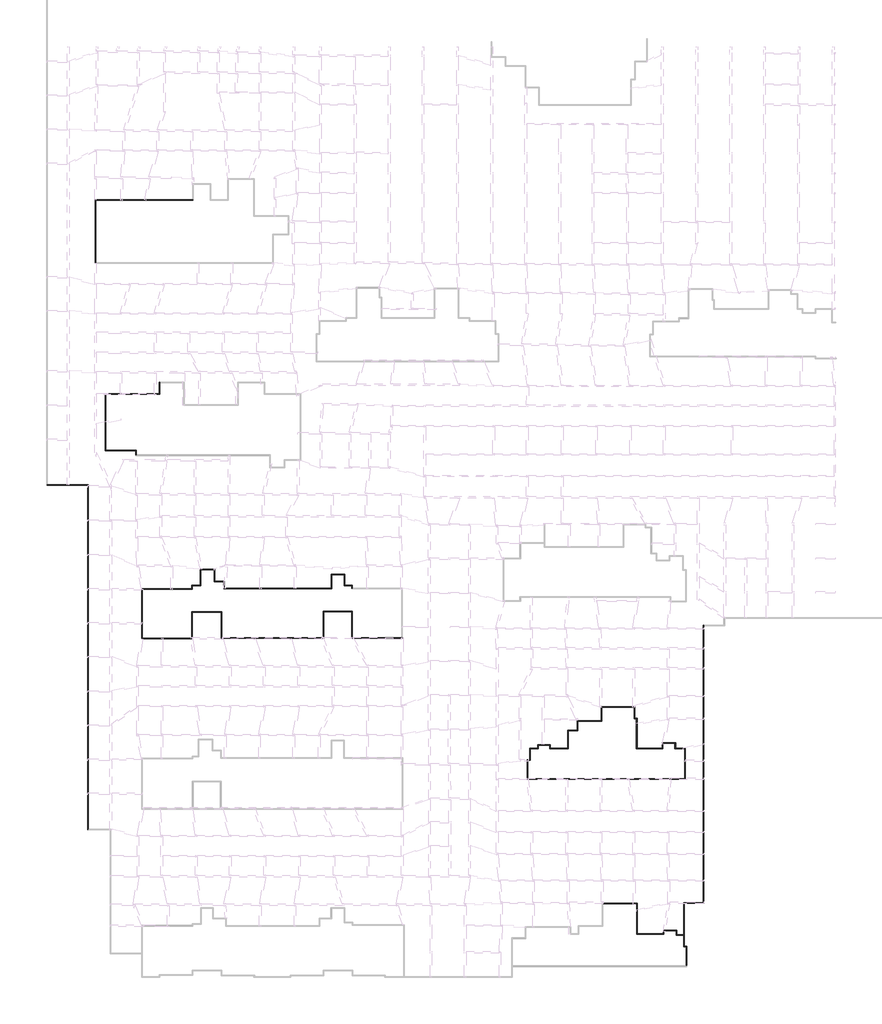
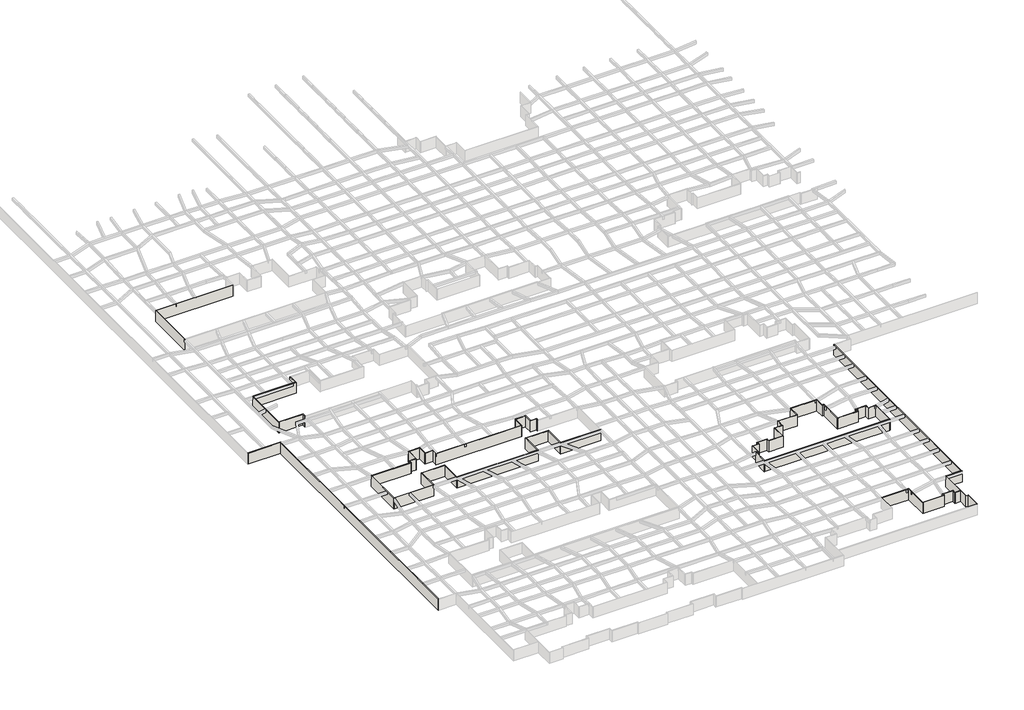
# One storey, part 2 of 45: 69 walls.
"""IFC4 building model written with IfcOpenShell, lengths in millimetres."""

from ifc_helpers import new_model, si_unit, origin, origin_with_axes, place, context, project, spatial, polyline, outline, extrude, faceted_brep, element, save

model = new_model("IFC4")

# Units and contexts
model_context = context("Model", 3, world=origin())
ifc_project = project(units=[si_unit("LENGTHUNIT", "METRE", prefix="MILLI")], contexts=[model_context])

# Site, building, storey
site = spatial("IfcSite", under=ifc_project)
building = spatial("IfcBuilding", under=site)
storey = spatial("IfcBuildingStorey", under=building, Name="户型图", Elevation=0.0)

# Walls
placement = place(None, origin())
element("IfcWall", 1, ObjectType="所有墙体", at=placement, inside=storey, context=model_context, shape_type="Brep", body=[
    faceted_brep([(-154980.5216564, -79588.0123265, 0.0), (-145700.5216564, -79588.0123265, 0.0), (-145580.5216564, -79588.0123265, 0.0), (-145580.5216564, -79588.0123265, 3300.0), (-145700.5216564, -79588.0123265, 3300.0), (-154980.5216564, -79588.0123265, 3300.0), (-154980.5216564, -79468.0123265, 0.0), (-154980.5216564, -79468.0123265, 3300.0), (-145580.5216564, -79468.0123265, 3300.0), (-145580.5216564, -79468.0123265, 0.0)], [[[0, 1, 2, 3, 4, 5]], [[6, 7, 8, 9]], [[2, 1, 0, 6, 9]], [[5, 4, 3, 8, 7]], [[0, 5, 7, 6]], [[3, 2, 9, 8]]]),
])
element("IfcWall", 2, ObjectType="所有墙体", at=placement, inside=storey, context=model_context, shape_type="Brep", body=[
    faceted_brep([(-145700.5216564, -79588.0123265, 0.0), (-145700.5216564, -158288.0123265, 0.0), (-145700.5216564, -158288.0123265, 3300.0), (-145700.5216564, -79588.0123265, 3300.0), (-145580.5216564, -79588.0123265, 0.0), (-145580.5216564, -79588.0123265, 3300.0), (-145580.5216564, -158168.0123265, 3300.0), (-145580.5216564, -158288.0123265, 3300.0), (-145580.5216564, -158288.0123265, 0.0), (-145580.5216564, -158168.0123265, 0.0)], [[[0, 1, 2, 3]], [[4, 5, 6, 7, 8, 9]], [[1, 0, 4, 9, 8]], [[3, 2, 7, 6, 5]], [[0, 3, 5, 4]], [[2, 1, 8, 7]]]),
])
element("IfcWall", 3, ObjectType="所有墙体", at=placement, inside=storey, context=model_context, shape_type="Brep", body=[
    faceted_brep([(-8780.5216564, -189468.0123265, 0.0), (-8780.5216564, -184968.0123265, 0.0), (-8780.5216564, -184968.0123265, 3300.0), (-8780.5216564, -189468.0123265, 3300.0), (-8900.5216564, -189468.0123265, 0.0), (-8900.5216564, -189468.0123265, 3300.0), (-8900.5216564, -185088.0123265, 3300.0), (-8900.5216564, -184968.0123265, 3300.0), (-8900.5216564, -184968.0123265, 0.0), (-8900.5216564, -185088.0123265, 0.0)], [[[0, 1, 2, 3]], [[4, 5, 6, 7, 8, 9]], [[1, 0, 4, 9, 8]], [[3, 2, 7, 6, 5]], [[0, 3, 5, 4]], [[2, 1, 8, 7]]]),
])
element("IfcWall", 4, ObjectType="所有墙体", at=placement, inside=storey, context=model_context, shape_type="Brep", body=[
    faceted_brep([(-8900.5216564, -184968.0123265, 0.0), (-9380.5216564, -184968.0123265, 0.0), (-9500.5216564, -184968.0123265, 0.0), (-9500.5216564, -184968.0123265, 3300.0), (-9380.5216564, -184968.0123265, 3300.0), (-8900.5216564, -184968.0123265, 3300.0), (-8900.5216564, -185088.0123265, 0.0), (-8900.5216564, -185088.0123265, 3300.0), (-9500.5216564, -185088.0123265, 3300.0), (-9500.5216564, -185088.0123265, 0.0)], [[[0, 1, 2, 3, 4, 5]], [[6, 7, 8, 9]], [[2, 1, 0, 6, 9]], [[5, 4, 3, 8, 7]], [[0, 5, 7, 6]], [[3, 2, 9, 8]]]),
])
element("IfcWall", 5, ObjectType="所有墙体", at=placement, inside=storey, context=model_context, shape_type="Brep", body=[
    faceted_brep([(-9380.5216564, -184968.0123265, 0.0), (-9380.5216564, -175188.0123265, 0.0), (-9380.5216564, -175068.0123265, 0.0), (-9380.5216564, -175068.0123265, 3300.0), (-9380.5216564, -175188.0123265, 3300.0), (-9380.5216564, -184968.0123265, 3300.0), (-9500.5216564, -184968.0123265, 0.0), (-9500.5216564, -184968.0123265, 3300.0), (-9500.5216564, -182430.9342179, 3300.0), (-9500.5216564, -182310.9342179, 3300.0), (-9500.5216564, -175068.0123265, 3300.0), (-9500.5216564, -175068.0123265, 0.0), (-9500.5216564, -182310.9342179, 0.0), (-9500.5216564, -182430.9342179, 0.0)], [[[0, 1, 2, 3, 4, 5]], [[6, 7, 8, 9, 10, 11, 12, 13]], [[2, 1, 0, 6, 13, 12, 11]], [[5, 4, 3, 10, 9, 8, 7]], [[0, 5, 7, 6]], [[3, 2, 11, 10]]]),
])
element("IfcWall", 6, ObjectType="所有墙体", at=placement, inside=storey, context=model_context, shape_type="Brep", body=[
    faceted_brep([(-9380.5216564, -175188.0123265, 0.0), (-4880.5216564, -175188.0123265, 0.0), (-4880.5216564, -175188.0123265, 3300.0), (-9380.5216564, -175188.0123265, 3300.0), (-9380.5216564, -175068.0123265, 0.0), (-9380.5216564, -175068.0123265, 3300.0), (-5000.5216564, -175068.0123265, 3300.0), (-4880.5216564, -175068.0123265, 3300.0), (-4880.5216564, -175068.0123265, 0.0), (-5000.5216564, -175068.0123265, 0.0)], [[[0, 1, 2, 3]], [[4, 5, 6, 7, 8, 9]], [[1, 0, 4, 9, 8]], [[3, 2, 7, 6, 5]], [[0, 3, 5, 4]], [[2, 1, 8, 7]]]),
])
element("IfcWall", 7, ObjectType="所有墙体", at=placement, inside=storey, context=model_context, shape_type="Brep", body=[
    faceted_brep([(-4880.5216564, -175068.0123265, 0.0), (-4880.5216564, -111688.0123265, 0.0), (-4880.5216564, -111568.0123265, 0.0), (-4880.5216564, -111568.0123265, 3300.0), (-4880.5216564, -111688.0123265, 3300.0), (-4880.5216564, -175068.0123265, 3300.0), (-5000.5216564, -175068.0123265, 0.0), (-5000.5216564, -175068.0123265, 3300.0), (-5000.5216564, -111568.0123265, 3300.0), (-5000.5216564, -111568.0123265, 0.0)], [[[0, 1, 2, 3, 4, 5]], [[6, 7, 8, 9]], [[2, 1, 0, 6, 9]], [[5, 4, 3, 8, 7]], [[0, 5, 7, 6]], [[3, 2, 9, 8]]]),
])
element("IfcWall", 8, ObjectType="所有墙体", at=placement, inside=storey, context=model_context, shape_type="Brep", body=[
    faceted_brep([(-27951.0528269, -175221.8863426, 0.0), (-20271.0528269, -175221.8863426, 0.0), (-20151.0528269, -175221.8863426, 0.0), (-20151.0528269, -175221.8863426, 3300.0), (-20271.0528269, -175221.8863426, 3300.0), (-27951.0528269, -175221.8863426, 3300.0), (-27951.0528269, -175101.8863426, 0.0), (-27951.0528269, -175101.8863426, 3300.0), (-20151.0528269, -175101.8863426, 3300.0), (-20151.0528269, -175101.8863426, 0.0)], [[[0, 1, 2, 3, 4, 5]], [[6, 7, 8, 9]], [[2, 1, 0, 6, 9]], [[5, 4, 3, 8, 7]], [[0, 5, 7, 6]], [[3, 2, 9, 8]]]),
])
element("IfcWall", 9, ObjectType="所有墙体", at=placement, inside=storey, context=model_context, shape_type="Brep", body=[
    faceted_brep([(-20271.0528269, -175221.8863426, 0.0), (-20271.0528269, -182221.8863426, 0.0), (-20271.0528269, -182221.8863426, 3300.0), (-20271.0528269, -175221.8863426, 3300.0), (-20151.0528269, -175221.8863426, 0.0), (-20151.0528269, -175221.8863426, 3300.0), (-20151.0528269, -182101.8863426, 3300.0), (-20151.0528269, -182221.8863426, 3300.0), (-20151.0528269, -182221.8863426, 0.0), (-20151.0528269, -182101.8863426, 0.0)], [[[0, 1, 2, 3]], [[4, 5, 6, 7, 8, 9]], [[1, 0, 4, 9, 8]], [[3, 2, 7, 6, 5]], [[0, 3, 5, 4]], [[2, 1, 8, 7]]]),
])
element("IfcWall", 10, ObjectType="所有墙体", at=placement, inside=storey, context=model_context, shape_type="Brep", body=[
    faceted_brep([(-20151.0528269, -182221.8863426, 0.0), (-14051.0528269, -182221.8863426, 0.0), (-14051.0528269, -182221.8863426, 3300.0), (-20151.0528269, -182221.8863426, 3300.0), (-20151.0528269, -182101.8863426, 0.0), (-20151.0528269, -182101.8863426, 3300.0), (-14171.0528269, -182101.8863426, 3300.0), (-14051.0528269, -182101.8863426, 3300.0), (-14051.0528269, -182101.8863426, 0.0), (-14171.0528269, -182101.8863426, 0.0)], [[[0, 1, 2, 3]], [[4, 5, 6, 7, 8, 9]], [[1, 0, 4, 9, 8]], [[3, 2, 7, 6, 5]], [[0, 3, 5, 4]], [[2, 1, 8, 7]]]),
])
element("IfcWall", 11, ObjectType="所有墙体", at=placement, inside=storey, context=model_context, shape_type="Brep", body=[
    faceted_brep([(-14051.0528269, -182101.8863426, 0.0), (-14051.0528269, -181430.9342179, 0.0), (-14051.0528269, -181310.9342179, 0.0), (-14051.0528269, -181310.9342179, 3300.0), (-14051.0528269, -181430.9342179, 3300.0), (-14051.0528269, -182101.8863426, 3300.0), (-14171.0528269, -182101.8863426, 0.0), (-14171.0528269, -182101.8863426, 3300.0), (-14171.0528269, -181310.9342179, 3300.0), (-14171.0528269, -181310.9342179, 0.0)], [[[0, 1, 2, 3, 4, 5]], [[6, 7, 8, 9]], [[2, 1, 0, 6, 9]], [[5, 4, 3, 8, 7]], [[0, 5, 7, 6]], [[3, 2, 9, 8]]]),
])
element("IfcWall", 12, ObjectType="所有墙体", at=placement, inside=storey, context=model_context, shape_type="Brep", body=[
    faceted_brep([(-14051.0528269, -181430.9342179, 0.0), (-11171.0528269, -181430.9342179, 0.0), (-11051.0528269, -181430.9342179, 0.0), (-11051.0528269, -181430.9342179, 3300.0), (-11171.0528269, -181430.9342179, 3300.0), (-14051.0528269, -181430.9342179, 3300.0), (-14051.0528269, -181310.9342179, 0.0), (-14051.0528269, -181310.9342179, 3300.0), (-11051.0528269, -181310.9342179, 3300.0), (-11051.0528269, -181310.9342179, 0.0)], [[[0, 1, 2, 3, 4, 5]], [[6, 7, 8, 9]], [[2, 1, 0, 6, 9]], [[5, 4, 3, 8, 7]], [[0, 5, 7, 6]], [[3, 2, 9, 8]]]),
])
element("IfcWall", 13, ObjectType="所有墙体", at=placement, inside=storey, context=model_context, shape_type="Brep", body=[
    faceted_brep([(-11171.0528269, -181430.9342179, 0.0), (-11171.0528269, -182430.9342179, 0.0), (-11171.0528269, -182430.9342179, 3300.0), (-11171.0528269, -181430.9342179, 3300.0), (-11051.0528269, -181430.9342179, 0.0), (-11051.0528269, -181430.9342179, 3300.0), (-11051.0528269, -182310.9342179, 3300.0), (-11051.0528269, -182430.9342179, 3300.0), (-11051.0528269, -182430.9342179, 0.0), (-11051.0528269, -182310.9342179, 0.0)], [[[0, 1, 2, 3]], [[4, 5, 6, 7, 8, 9]], [[1, 0, 4, 9, 8]], [[3, 2, 7, 6, 5]], [[0, 3, 5, 4]], [[2, 1, 8, 7]]]),
])
element("IfcWall", 14, ObjectType="所有墙体", at=placement, inside=storey, context=model_context, shape_type="SweptSolid", body=[
    extrude(outline(polyline([(-9500.5216564, -182430.9342179), (-11051.0528269, -182430.9342179), (-11051.0528269, -182310.9342179), (-9500.5216564, -182310.9342179), (-9500.5216564, -182430.9342179)])), origin_with_axes(), (0.0, 0.0, 1.0), 3300.0),
])
element("IfcWall", 15, ObjectType="所有墙体", at=placement, inside=storey, context=model_context, shape_type="Brep", body=[
    faceted_brep([(-133310.9438267, -103315.0953667, 0.0), (-133310.9438267, -114643.3262311, 0.0), (-133310.9438267, -114643.3262311, 3300.0), (-133310.9438267, -103315.0953667, 3300.0), (-133190.9438267, -103315.0953667, 0.0), (-133190.9438267, -103315.0953667, 3300.0), (-133190.9438267, -103435.0953667, 3300.0), (-133190.9438267, -114523.3262311, 3300.0), (-133190.9438267, -114643.3262311, 3300.0), (-133190.9438267, -114643.3262311, 0.0), (-133190.9438267, -114523.3262311, 0.0), (-133190.9438267, -103435.0953667, 0.0)], [[[0, 1, 2, 3]], [[4, 5, 6, 7, 8, 9, 10, 11]], [[1, 0, 4, 11, 10, 9]], [[3, 2, 8, 7, 6, 5]], [[2, 1, 9, 8]], [[0, 3, 5, 4]]]),
])
element("IfcWall", 16, ObjectType="所有墙体", at=placement, inside=storey, context=model_context, shape_type="Brep", body=[
    faceted_brep([(-133190.9438267, -114643.3262311, 0.0), (-121790.9438267, -114643.3262311, 0.0), (-121790.9438267, -114643.3262311, 3300.0), (-133190.9438267, -114643.3262311, 3300.0), (-133190.9438267, -114523.3262311, 0.0), (-133190.9438267, -114523.3262311, 3300.0), (-121910.9438267, -114523.3262311, 3300.0), (-121790.9438267, -114523.3262311, 3300.0), (-121790.9438267, -114523.3262311, 0.0), (-121910.9438267, -114523.3262311, 0.0)], [[[0, 1, 2, 3]], [[4, 5, 6, 7, 8, 9]], [[1, 0, 4, 9, 8]], [[3, 2, 7, 6, 5]], [[0, 3, 5, 4]], [[2, 1, 8, 7]]]),
])
element("IfcWall", 17, ObjectType="所有墙体", at=placement, inside=storey, context=model_context, shape_type="Brep", body=[
    faceted_brep([(-121790.9438267, -114523.3262311, 0.0), (-121790.9438267, -108643.3262311, 0.0), (-121790.9438267, -108523.3262311, 0.0), (-121790.9438267, -108523.3262311, 3300.0), (-121790.9438267, -108643.3262311, 3300.0), (-121790.9438267, -114523.3262311, 3300.0), (-121910.9438267, -114523.3262311, 0.0), (-121910.9438267, -114523.3262311, 3300.0), (-121910.9438267, -108523.3262311, 3300.0), (-121910.9438267, -108523.3262311, 0.0)], [[[0, 1, 2, 3, 4, 5]], [[6, 7, 8, 9]], [[2, 1, 0, 6, 9]], [[5, 4, 3, 8, 7]], [[0, 5, 7, 6]], [[3, 2, 9, 8]]]),
])
element("IfcWall", 18, ObjectType="所有墙体", at=placement, inside=storey, context=model_context, shape_type="Brep", body=[
    faceted_brep([(-121790.9438267, -108643.3262311, 0.0), (-115210.9438267, -108643.3262311, 0.0), (-115090.9438267, -108643.3262311, 0.0), (-115090.9438267, -108643.3262311, 3300.0), (-115210.9438267, -108643.3262311, 3300.0), (-121790.9438267, -108643.3262311, 3300.0), (-121790.9438267, -108523.3262311, 0.0), (-121790.9438267, -108523.3262311, 3300.0), (-115090.9438267, -108523.3262311, 3300.0), (-115090.9438267, -108523.3262311, 0.0)], [[[0, 1, 2, 3, 4, 5]], [[6, 7, 8, 9]], [[2, 1, 0, 6, 9]], [[5, 4, 3, 8, 7]], [[0, 5, 7, 6]], [[3, 2, 9, 8]]]),
])
element("IfcWall", 19, ObjectType="所有墙体", at=placement, inside=storey, context=model_context, shape_type="Brep", body=[
    faceted_brep([(-115210.9438267, -108643.3262311, 0.0), (-115210.9438267, -114616.2273817, 0.0), (-115210.9438267, -114616.2273817, 3300.0), (-115210.9438267, -108643.3262311, 3300.0), (-115090.9438267, -108643.3262311, 0.0), (-115090.9438267, -108643.3262311, 3300.0), (-115090.9438267, -114496.2273817, 3300.0), (-115090.9438267, -114616.2273817, 3300.0), (-115090.9438267, -114616.2273817, 0.0), (-115090.9438267, -114496.2273817, 0.0)], [[[0, 1, 2, 3]], [[4, 5, 6, 7, 8, 9]], [[1, 0, 4, 9, 8]], [[3, 2, 7, 6, 5]], [[0, 3, 5, 4]], [[2, 1, 8, 7]]]),
])
element("IfcWall", 20, ObjectType="所有墙体", at=placement, inside=storey, context=model_context, shape_type="Brep", body=[
    faceted_brep([(-115090.9438267, -114616.2273817, 0.0), (-91790.9438267, -114616.2273817, 0.0), (-91790.9438267, -114616.2273817, 3300.0), (-115090.9438267, -114616.2273817, 3300.0), (-115090.9438267, -114496.2273817, 0.0), (-115090.9438267, -114496.2273817, 3300.0), (-91910.9438267, -114496.2273817, 3300.0), (-91790.9438267, -114496.2273817, 3300.0), (-91790.9438267, -114496.2273817, 0.0), (-91910.9438267, -114496.2273817, 0.0)], [[[0, 1, 2, 3]], [[4, 5, 6, 7, 8, 9]], [[1, 0, 4, 9, 8]], [[3, 2, 7, 6, 5]], [[0, 3, 5, 4]], [[2, 1, 8, 7]]]),
])
element("IfcWall", 21, ObjectType="所有墙体", at=placement, inside=storey, context=model_context, shape_type="Brep", body=[
    faceted_brep([(-91790.9438267, -114496.2273817, 0.0), (-91790.9438267, -108516.2273817, 0.0), (-91790.9438267, -108396.2273817, 0.0), (-91790.9438267, -108396.2273817, 3300.0), (-91790.9438267, -108516.2273817, 3300.0), (-91790.9438267, -114496.2273817, 3300.0), (-91910.9438267, -114496.2273817, 0.0), (-91910.9438267, -114496.2273817, 3300.0), (-91910.9438267, -108396.2273817, 3300.0), (-91910.9438267, -108396.2273817, 0.0)], [[[0, 1, 2, 3, 4, 5]], [[6, 7, 8, 9]], [[2, 1, 0, 6, 9]], [[5, 4, 3, 8, 7]], [[0, 5, 7, 6]], [[3, 2, 9, 8]]]),
])
element("IfcWall", 22, ObjectType="所有墙体", at=placement, inside=storey, context=model_context, shape_type="Brep", body=[
    faceted_brep([(-91790.9438267, -108516.2273817, 0.0), (-85410.9438267, -108516.2273817, 0.0), (-85290.9438267, -108516.2273817, 0.0), (-85290.9438267, -108516.2273817, 3300.0), (-85410.9438267, -108516.2273817, 3300.0), (-91790.9438267, -108516.2273817, 3300.0), (-91790.9438267, -108396.2273817, 0.0), (-91790.9438267, -108396.2273817, 3300.0), (-85290.9438267, -108396.2273817, 3300.0), (-85290.9438267, -108396.2273817, 0.0)], [[[0, 1, 2, 3, 4, 5]], [[6, 7, 8, 9]], [[2, 1, 0, 6, 9]], [[5, 4, 3, 8, 7]], [[0, 5, 7, 6]], [[3, 2, 9, 8]]]),
])
element("IfcWall", 23, ObjectType="所有墙体", at=placement, inside=storey, context=model_context, shape_type="Brep", body=[
    faceted_brep([(-85410.9438267, -108516.2273817, 0.0), (-85410.9438267, -114616.2273817, 0.0), (-85410.9438267, -114616.2273817, 3300.0), (-85410.9438267, -108516.2273817, 3300.0), (-85290.9438267, -108516.2273817, 0.0), (-85290.9438267, -108516.2273817, 3300.0), (-85290.9438267, -114496.2273817, 3300.0), (-85290.9438267, -114616.2273817, 3300.0), (-85290.9438267, -114616.2273817, 0.0), (-85290.9438267, -114496.2273817, 0.0)], [[[0, 1, 2, 3]], [[4, 5, 6, 7, 8, 9]], [[1, 0, 4, 9, 8]], [[3, 2, 7, 6, 5]], [[0, 3, 5, 4]], [[2, 1, 8, 7]]]),
])
element("IfcWall", 24, ObjectType="所有墙体", at=placement, inside=storey, context=model_context, shape_type="Brep", body=[
    faceted_brep([(-85290.9438267, -114616.2273817, 0.0), (-73790.9438267, -114616.2273817, 0.0), (-73790.9438267, -114616.2273817, 3300.0), (-85290.9438267, -114616.2273817, 3300.0), (-85290.9438267, -114496.2273817, 0.0), (-85290.9438267, -114496.2273817, 3300.0), (-73910.9438267, -114496.2273817, 3300.0), (-73790.9438267, -114496.2273817, 3300.0), (-73790.9438267, -114496.2273817, 0.0), (-73910.9438267, -114496.2273817, 0.0)], [[[0, 1, 2, 3]], [[4, 5, 6, 7, 8, 9]], [[1, 0, 4, 9, 8]], [[3, 2, 7, 6, 5]], [[0, 3, 5, 4]], [[2, 1, 8, 7]]]),
])
element("IfcWall", 25, ObjectType="所有墙体", at=placement, inside=storey, context=model_context, shape_type="Brep", body=[
    faceted_brep([(-85290.9438267, -103096.2273817, 0.0), (-85290.9438267, -102496.2273817, 0.0), (-85290.9438267, -102496.2273817, 3300.0), (-85290.9438267, -103096.2273817, 3300.0), (-85410.9438267, -103096.2273817, 0.0), (-85410.9438267, -103096.2273817, 3300.0), (-85410.9438267, -102616.2273817, 3300.0), (-85410.9438267, -102496.2273817, 3300.0), (-85410.9438267, -102496.2273817, 0.0), (-85410.9438267, -102616.2273817, 0.0)], [[[0, 1, 2, 3]], [[4, 5, 6, 7, 8, 9]], [[1, 0, 4, 9, 8]], [[3, 2, 7, 6, 5]], [[0, 3, 5, 4]], [[2, 1, 8, 7]]]),
])
element("IfcWall", 26, ObjectType="所有墙体", at=placement, inside=storey, context=model_context, shape_type="Brep", body=[
    faceted_brep([(-85410.9438267, -102496.2273817, 0.0), (-86990.9438267, -102496.2273817, 0.0), (-87110.9438267, -102496.2273817, 0.0), (-87110.9438267, -102496.2273817, 3300.0), (-86990.9438267, -102496.2273817, 3300.0), (-85410.9438267, -102496.2273817, 3300.0), (-85410.9438267, -102616.2273817, 0.0), (-85410.9438267, -102616.2273817, 3300.0), (-87110.9438267, -102616.2273817, 3300.0), (-87110.9438267, -102616.2273817, 0.0)], [[[0, 1, 2, 3, 4, 5]], [[6, 7, 8, 9]], [[2, 1, 0, 6, 9]], [[5, 4, 3, 8, 7]], [[0, 5, 7, 6]], [[3, 2, 9, 8]]]),
])
element("IfcWall", 27, ObjectType="所有墙体", at=placement, inside=storey, context=model_context, shape_type="Brep", body=[
    faceted_brep([(-86990.9438267, -102496.2273817, 0.0), (-86990.9438267, -99996.2273817, 0.0), (-86990.9438267, -99996.2273817, 3300.0), (-86990.9438267, -102496.2273817, 3300.0), (-87110.9438267, -102496.2273817, 0.0), (-87110.9438267, -102496.2273817, 3300.0), (-87110.9438267, -100116.2273817, 3300.0), (-87110.9438267, -99996.2273817, 3300.0), (-87110.9438267, -99996.2273817, 0.0), (-87110.9438267, -100116.2273817, 0.0)], [[[0, 1, 2, 3]], [[4, 5, 6, 7, 8, 9]], [[1, 0, 4, 9, 8]], [[3, 2, 7, 6, 5]], [[0, 3, 5, 4]], [[2, 1, 8, 7]]]),
])
element("IfcWall", 28, ObjectType="所有墙体", at=placement, inside=storey, context=model_context, shape_type="Brep", body=[
    faceted_brep([(-87110.9438267, -99996.2273817, 0.0), (-90010.9438267, -99996.2273817, 0.0), (-90010.9438267, -99996.2273817, 3300.0), (-87110.9438267, -99996.2273817, 3300.0), (-87110.9438267, -100116.2273817, 0.0), (-87110.9438267, -100116.2273817, 3300.0), (-89890.9438267, -100116.2273817, 3300.0), (-90010.9438267, -100116.2273817, 3300.0), (-90010.9438267, -100116.2273817, 0.0), (-89890.9438267, -100116.2273817, 0.0)], [[[0, 1, 2, 3]], [[4, 5, 6, 7, 8, 9]], [[1, 0, 4, 9, 8]], [[3, 2, 7, 6, 5]], [[0, 3, 5, 4]], [[2, 1, 8, 7]]]),
])
element("IfcWall", 29, ObjectType="所有墙体", at=placement, inside=storey, context=model_context, shape_type="Brep", body=[
    faceted_brep([(-90010.9438267, -100116.2273817, 0.0), (-90010.9438267, -103096.2273817, 0.0), (-90010.9438267, -103216.2273817, 0.0), (-90010.9438267, -103216.2273817, 3300.0), (-90010.9438267, -103096.2273817, 3300.0), (-90010.9438267, -100116.2273817, 3300.0), (-89890.9438267, -100116.2273817, 0.0), (-89890.9438267, -100116.2273817, 3300.0), (-89890.9438267, -103216.2273817, 3300.0), (-89890.9438267, -103216.2273817, 0.0)], [[[0, 1, 2, 3, 4, 5]], [[6, 7, 8, 9]], [[2, 1, 0, 6, 9]], [[5, 4, 3, 8, 7]], [[0, 5, 7, 6]], [[3, 2, 9, 8]]]),
])
element("IfcWall", 30, ObjectType="所有墙体", at=placement, inside=storey, context=model_context, shape_type="Brep", body=[
    faceted_brep([(-90010.9438267, -103096.2273817, 0.0), (-114494.8894141, -103096.2273817, 0.0), (-114614.8894141, -103096.2273817, 0.0), (-114614.8894141, -103096.2273817, 3300.0), (-114494.8894141, -103096.2273817, 3300.0), (-90010.9438267, -103096.2273817, 3300.0), (-90010.9438267, -103216.2273817, 0.0), (-90010.9438267, -103216.2273817, 3300.0), (-114614.8894141, -103216.2273817, 3300.0), (-114614.8894141, -103216.2273817, 0.0)], [[[0, 1, 2, 3, 4, 5]], [[6, 7, 8, 9]], [[2, 1, 0, 6, 9]], [[5, 4, 3, 8, 7]], [[0, 5, 7, 6]], [[3, 2, 9, 8]]]),
])
element("IfcWall", 31, ObjectType="所有墙体", at=placement, inside=storey, context=model_context, shape_type="Brep", body=[
    faceted_brep([(-114494.8894141, -103096.2273817, 0.0), (-114494.8894141, -101496.2273817, 0.0), (-114494.8894141, -101496.2273817, 3300.0), (-114494.8894141, -103096.2273817, 3300.0), (-114614.8894141, -103096.2273817, 0.0), (-114614.8894141, -103096.2273817, 3300.0), (-114614.8894141, -101616.2273817, 3300.0), (-114614.8894141, -101496.2273817, 3300.0), (-114614.8894141, -101496.2273817, 0.0), (-114614.8894141, -101616.2273817, 0.0)], [[[0, 1, 2, 3]], [[4, 5, 6, 7, 8, 9]], [[1, 0, 4, 9, 8]], [[3, 2, 7, 6, 5]], [[0, 3, 5, 4]], [[2, 1, 8, 7]]]),
])
element("IfcWall", 32, ObjectType="所有墙体", at=placement, inside=storey, context=model_context, shape_type="Brep", body=[
    faceted_brep([(-114614.8894141, -101496.2273817, 0.0), (-116694.8894141, -101496.2273817, 0.0), (-116814.8894141, -101496.2273817, 0.0), (-116814.8894141, -101496.2273817, 3300.0), (-116694.8894141, -101496.2273817, 3300.0), (-114614.8894141, -101496.2273817, 3300.0), (-114614.8894141, -101616.2273817, 0.0), (-114614.8894141, -101616.2273817, 3300.0), (-116814.8894141, -101616.2273817, 3300.0), (-116814.8894141, -101616.2273817, 0.0)], [[[0, 1, 2, 3, 4, 5]], [[6, 7, 8, 9]], [[2, 1, 0, 6, 9]], [[5, 4, 3, 8, 7]], [[0, 5, 7, 6]], [[3, 2, 9, 8]]]),
])
element("IfcWall", 33, ObjectType="所有墙体", at=placement, inside=storey, context=model_context, shape_type="Brep", body=[
    faceted_brep([(-116694.8894141, -101496.2273817, 0.0), (-116694.8894141, -98815.2904885, 0.0), (-116694.8894141, -98815.2904885, 3300.0), (-116694.8894141, -101496.2273817, 3300.0), (-116814.8894141, -101496.2273817, 0.0), (-116814.8894141, -101496.2273817, 3300.0), (-116814.8894141, -98935.2904885, 3300.0), (-116814.8894141, -98815.2904885, 3300.0), (-116814.8894141, -98815.2904885, 0.0), (-116814.8894141, -98935.2904885, 0.0)], [[[0, 1, 2, 3]], [[4, 5, 6, 7, 8, 9]], [[1, 0, 4, 9, 8]], [[3, 2, 7, 6, 5]], [[0, 3, 5, 4]], [[2, 1, 8, 7]]]),
])
element("IfcWall", 34, ObjectType="所有墙体", at=placement, inside=storey, context=model_context, shape_type="Brep", body=[
    faceted_brep([(-116814.8894141, -98815.2904885, 0.0), (-120017.441353, -98815.2904885, 0.0), (-120017.441353, -98815.2904885, 3300.0), (-116814.8894141, -98815.2904885, 3300.0), (-116814.8894141, -98935.2904885, 0.0), (-116814.8894141, -98935.2904885, 3300.0), (-119897.441353, -98935.2904885, 3300.0), (-120017.441353, -98935.2904885, 3300.0), (-120017.441353, -98935.2904885, 0.0), (-119897.441353, -98935.2904885, 0.0)], [[[0, 1, 2, 3]], [[4, 5, 6, 7, 8, 9]], [[1, 0, 4, 9, 8]], [[3, 2, 7, 6, 5]], [[0, 3, 5, 4]], [[2, 1, 8, 7]]]),
])
element("IfcWall", 35, ObjectType="所有墙体", at=placement, inside=storey, context=model_context, shape_type="Brep", body=[
    faceted_brep([(-120017.441353, -98935.2904885, 0.0), (-120017.441353, -102496.2273817, 0.0), (-120017.441353, -102616.2273817, 0.0), (-120017.441353, -102616.2273817, 3300.0), (-120017.441353, -102496.2273817, 3300.0), (-120017.441353, -98935.2904885, 3300.0), (-119897.441353, -98935.2904885, 0.0), (-119897.441353, -98935.2904885, 3300.0), (-119897.441353, -102616.2273817, 3300.0), (-119897.441353, -102616.2273817, 0.0)], [[[0, 1, 2, 3, 4, 5]], [[6, 7, 8, 9]], [[2, 1, 0, 6, 9]], [[5, 4, 3, 8, 7]], [[0, 5, 7, 6]], [[3, 2, 9, 8]]]),
])
element("IfcWall", 36, ObjectType="所有墙体", at=placement, inside=storey, context=model_context, shape_type="Brep", body=[
    faceted_brep([(-120017.441353, -102496.2273817, 0.0), (-121910.9438267, -102496.2273817, 0.0), (-121910.9438267, -102496.2273817, 3300.0), (-120017.441353, -102496.2273817, 3300.0), (-120017.441353, -102616.2273817, 0.0), (-120017.441353, -102616.2273817, 3300.0), (-121790.9438267, -102616.2273817, 3300.0), (-121910.9438267, -102616.2273817, 3300.0), (-121910.9438267, -102616.2273817, 0.0), (-121790.9438267, -102616.2273817, 0.0)], [[[0, 1, 2, 3]], [[4, 5, 6, 7, 8, 9]], [[1, 0, 4, 9, 8]], [[3, 2, 7, 6, 5]], [[0, 3, 5, 4]], [[2, 1, 8, 7]]]),
])
element("IfcWall", 37, ObjectType="所有墙体", at=placement, inside=storey, context=model_context, shape_type="Brep", body=[
    faceted_brep([(-121910.9438267, -102616.2273817, 0.0), (-121910.9438267, -103315.0953667, 0.0), (-121910.9438267, -103435.0953667, 0.0), (-121910.9438267, -103435.0953667, 3300.0), (-121910.9438267, -103315.0953667, 3300.0), (-121910.9438267, -102616.2273817, 3300.0), (-121790.9438267, -102616.2273817, 0.0), (-121790.9438267, -102616.2273817, 3300.0), (-121790.9438267, -103435.0953667, 3300.0), (-121790.9438267, -103435.0953667, 0.0)], [[[0, 1, 2, 3, 4, 5]], [[6, 7, 8, 9]], [[2, 1, 0, 6, 9]], [[5, 4, 3, 8, 7]], [[0, 5, 7, 6]], [[3, 2, 9, 8]]]),
])
element("IfcWall", 38, ObjectType="所有墙体", at=placement, inside=storey, context=model_context, shape_type="SweptSolid", body=[
    extrude(outline(polyline([(-133190.9438267, -103315.0953667), (-121910.9438267, -103315.0953667), (-121910.9438267, -103435.0953667), (-133190.9438267, -103435.0953667), (-133190.9438267, -103315.0953667)])), origin_with_axes(), (0.0, 0.0, 1.0), 3300.0),
])
element("IfcWall", 39, ObjectType="所有墙体", at=placement, inside=storey, context=model_context, shape_type="Brep", body=[
    faceted_brep([(-45189.2481784, -146753.3401094, 0.0), (-45189.2481784, -146633.3401094, 0.0), (-45189.2481784, -142491.0431969, 0.0), (-45189.2481784, -142371.0431969, 0.0), (-45189.2481784, -142371.0431969, 3300.0), (-45189.2481784, -142491.0431969, 3300.0), (-45189.2481784, -146633.3401094, 3300.0), (-45189.2481784, -146753.3401094, 3300.0), (-45309.2481784, -146753.3401094, 0.0), (-45309.2481784, -146753.3401094, 3300.0), (-45309.2481784, -142371.0431969, 3300.0), (-45309.2481784, -142371.0431969, 0.0)], [[[0, 1, 2, 3, 4, 5, 6, 7]], [[8, 9, 10, 11]], [[3, 2, 1, 0, 8, 11]], [[7, 6, 5, 4, 10, 9]], [[4, 3, 11, 10]], [[0, 7, 9, 8]]]),
])
element("IfcWall", 40, ObjectType="所有墙体", at=placement, inside=storey, context=model_context, shape_type="Brep", body=[
    faceted_brep([(-45189.2481784, -142491.0431969, 0.0), (-44589.2481784, -142491.0431969, 0.0), (-44589.2481784, -142491.0431969, 3300.0), (-45189.2481784, -142491.0431969, 3300.0), (-45189.2481784, -142371.0431969, 0.0), (-45189.2481784, -142371.0431969, 3300.0), (-44709.2481784, -142371.0431969, 3300.0), (-44589.2481784, -142371.0431969, 3300.0), (-44589.2481784, -142371.0431969, 0.0), (-44709.2481784, -142371.0431969, 0.0)], [[[0, 1, 2, 3]], [[4, 5, 6, 7, 8, 9]], [[1, 0, 4, 9, 8]], [[3, 2, 7, 6, 5]], [[0, 3, 5, 4]], [[2, 1, 8, 7]]]),
])
element("IfcWall", 41, ObjectType="所有墙体", at=placement, inside=storey, context=model_context, shape_type="Brep", body=[
    faceted_brep([(-44589.2481784, -142371.0431969, 0.0), (-44589.2481784, -139791.0431969, 0.0), (-44589.2481784, -139671.0431969, 0.0), (-44589.2481784, -139671.0431969, 3300.0), (-44589.2481784, -139791.0431969, 3300.0), (-44589.2481784, -142371.0431969, 3300.0), (-44709.2481784, -142371.0431969, 0.0), (-44709.2481784, -142371.0431969, 3300.0), (-44709.2481784, -139671.0431969, 3300.0), (-44709.2481784, -139671.0431969, 0.0)], [[[0, 1, 2, 3, 4, 5]], [[6, 7, 8, 9]], [[2, 1, 0, 6, 9]], [[5, 4, 3, 8, 7]], [[0, 5, 7, 6]], [[3, 2, 9, 8]]]),
])
element("IfcWall", 42, ObjectType="所有墙体", at=placement, inside=storey, context=model_context, shape_type="Brep", body=[
    faceted_brep([(-44589.2481784, -139791.0431969, 0.0), (-42789.2481784, -139791.0431969, 0.0), (-42789.2481784, -139791.0431969, 3300.0), (-44589.2481784, -139791.0431969, 3300.0), (-44589.2481784, -139671.0431969, 0.0), (-44589.2481784, -139671.0431969, 3300.0), (-42909.2481784, -139671.0431969, 3300.0), (-42789.2481784, -139671.0431969, 3300.0), (-42789.2481784, -139671.0431969, 0.0), (-42909.2481784, -139671.0431969, 0.0)], [[[0, 1, 2, 3]], [[4, 5, 6, 7, 8, 9]], [[1, 0, 4, 9, 8]], [[3, 2, 7, 6, 5]], [[0, 3, 5, 4]], [[2, 1, 8, 7]]]),
])
element("IfcWall", 43, ObjectType="所有墙体", at=placement, inside=storey, context=model_context, shape_type="Brep", body=[
    faceted_brep([(-42789.2481784, -139671.0431969, 0.0), (-42789.2481784, -138991.0431969, 0.0), (-42789.2481784, -138871.0431969, 0.0), (-42789.2481784, -138871.0431969, 3300.0), (-42789.2481784, -138991.0431969, 3300.0), (-42789.2481784, -139671.0431969, 3300.0), (-42909.2481784, -139671.0431969, 0.0), (-42909.2481784, -139671.0431969, 3300.0), (-42909.2481784, -138871.0431969, 3300.0), (-42909.2481784, -138871.0431969, 0.0)], [[[0, 1, 2, 3, 4, 5]], [[6, 7, 8, 9]], [[2, 1, 0, 6, 9]], [[5, 4, 3, 8, 7]], [[0, 5, 7, 6]], [[3, 2, 9, 8]]]),
])
element("IfcWall", 44, ObjectType="所有墙体", at=placement, inside=storey, context=model_context, shape_type="Brep", body=[
    faceted_brep([(-42789.2481784, -138991.0431969, 0.0), (-40109.2481784, -138991.0431969, 0.0), (-39989.2481784, -138991.0431969, 0.0), (-39989.2481784, -138991.0431969, 3300.0), (-40109.2481784, -138991.0431969, 3300.0), (-42789.2481784, -138991.0431969, 3300.0), (-42789.2481784, -138871.0431969, 0.0), (-42789.2481784, -138871.0431969, 3300.0), (-39989.2481784, -138871.0431969, 3300.0), (-39989.2481784, -138871.0431969, 0.0)], [[[0, 1, 2, 3, 4, 5]], [[6, 7, 8, 9]], [[2, 1, 0, 6, 9]], [[5, 4, 3, 8, 7]], [[0, 5, 7, 6]], [[3, 2, 9, 8]]]),
])
element("IfcWall", 45, ObjectType="所有墙体", at=placement, inside=storey, context=model_context, shape_type="Brep", body=[
    faceted_brep([(-40109.2481784, -138991.0431969, 0.0), (-40109.2481784, -139791.0431969, 0.0), (-40109.2481784, -139791.0431969, 3300.0), (-40109.2481784, -138991.0431969, 3300.0), (-39989.2481784, -138991.0431969, 0.0), (-39989.2481784, -138991.0431969, 3300.0), (-39989.2481784, -139671.0431969, 3300.0), (-39989.2481784, -139791.0431969, 3300.0), (-39989.2481784, -139791.0431969, 0.0), (-39989.2481784, -139671.0431969, 0.0)], [[[0, 1, 2, 3]], [[4, 5, 6, 7, 8, 9]], [[1, 0, 4, 9, 8]], [[3, 2, 7, 6, 5]], [[0, 3, 5, 4]], [[2, 1, 8, 7]]]),
])
element("IfcWall", 46, ObjectType="所有墙体", at=placement, inside=storey, context=model_context, shape_type="Brep", body=[
    faceted_brep([(-39989.2481784, -139791.0431969, 0.0), (-35889.2481784, -139791.0431969, 0.0), (-35889.2481784, -139791.0431969, 3300.0), (-39989.2481784, -139791.0431969, 3300.0), (-39989.2481784, -139671.0431969, 0.0), (-39989.2481784, -139671.0431969, 3300.0), (-36009.2481784, -139671.0431969, 3300.0), (-35889.2481784, -139671.0431969, 3300.0), (-35889.2481784, -139671.0431969, 0.0), (-36009.2481784, -139671.0431969, 0.0)], [[[0, 1, 2, 3]], [[4, 5, 6, 7, 8, 9]], [[1, 0, 4, 9, 8]], [[3, 2, 7, 6, 5]], [[0, 3, 5, 4]], [[2, 1, 8, 7]]]),
])
element("IfcWall", 47, ObjectType="所有墙体", at=placement, inside=storey, context=model_context, shape_type="Brep", body=[
    faceted_brep([(-35889.2481784, -139671.0431969, 0.0), (-35889.2481784, -135691.0431969, 0.0), (-35889.2481784, -135571.0431969, 0.0), (-35889.2481784, -135571.0431969, 3300.0), (-35889.2481784, -135691.0431969, 3300.0), (-35889.2481784, -139671.0431969, 3300.0), (-36009.2481784, -139671.0431969, 0.0), (-36009.2481784, -139671.0431969, 3300.0), (-36009.2481784, -135571.0431969, 3300.0), (-36009.2481784, -135571.0431969, 0.0)], [[[0, 1, 2, 3, 4, 5]], [[6, 7, 8, 9]], [[2, 1, 0, 6, 9]], [[5, 4, 3, 8, 7]], [[0, 5, 7, 6]], [[3, 2, 9, 8]]]),
])
element("IfcWall", 48, ObjectType="所有墙体", at=placement, inside=storey, context=model_context, shape_type="Brep", body=[
    faceted_brep([(-35889.2481784, -135691.0431969, 0.0), (-33689.2481784, -135691.0431969, 0.0), (-33689.2481784, -135691.0431969, 3300.0), (-35889.2481784, -135691.0431969, 3300.0), (-35889.2481784, -135571.0431969, 0.0), (-35889.2481784, -135571.0431969, 3300.0), (-33809.2481784, -135571.0431969, 3300.0), (-33689.2481784, -135571.0431969, 3300.0), (-33689.2481784, -135571.0431969, 0.0), (-33809.2481784, -135571.0431969, 0.0)], [[[0, 1, 2, 3]], [[4, 5, 6, 7, 8, 9]], [[1, 0, 4, 9, 8]], [[3, 2, 7, 6, 5]], [[0, 3, 5, 4]], [[2, 1, 8, 7]]]),
])
element("IfcWall", 49, ObjectType="所有墙体", at=placement, inside=storey, context=model_context, shape_type="Brep", body=[
    faceted_brep([(-33689.2481784, -135571.0431969, 0.0), (-33689.2481784, -133547.4515368, 0.0), (-33689.2481784, -133427.4515368, 0.0), (-33689.2481784, -133427.4515368, 3300.0), (-33689.2481784, -133547.4515368, 3300.0), (-33689.2481784, -135571.0431969, 3300.0), (-33809.2481784, -135571.0431969, 0.0), (-33809.2481784, -135571.0431969, 3300.0), (-33809.2481784, -133427.4515368, 3300.0), (-33809.2481784, -133427.4515368, 0.0)], [[[0, 1, 2, 3, 4, 5]], [[6, 7, 8, 9]], [[2, 1, 0, 6, 9]], [[5, 4, 3, 8, 7]], [[0, 5, 7, 6]], [[3, 2, 9, 8]]]),
])
element("IfcWall", 50, ObjectType="所有墙体", at=placement, inside=storey, context=model_context, shape_type="Brep", body=[
    faceted_brep([(-33689.2481784, -133547.4515368, 0.0), (-28189.2481784, -133547.4515368, 0.0), (-28189.2481784, -133547.4515368, 3300.0), (-33689.2481784, -133547.4515368, 3300.0), (-33689.2481784, -133427.4515368, 0.0), (-33689.2481784, -133427.4515368, 3300.0), (-28309.2481784, -133427.4515368, 3300.0), (-28189.2481784, -133427.4515368, 3300.0), (-28189.2481784, -133427.4515368, 0.0), (-28309.2481784, -133427.4515368, 0.0)], [[[0, 1, 2, 3]], [[4, 5, 6, 7, 8, 9]], [[1, 0, 4, 9, 8]], [[3, 2, 7, 6, 5]], [[0, 3, 5, 4]], [[2, 1, 8, 7]]]),
])
element("IfcWall", 51, ObjectType="所有墙体", at=placement, inside=storey, context=model_context, shape_type="Brep", body=[
    faceted_brep([(-28189.2481784, -133427.4515368, 0.0), (-28189.2481784, -130299.7816616, 0.0), (-28189.2481784, -130179.7816616, 0.0), (-28189.2481784, -130179.7816616, 3300.0), (-28189.2481784, -130299.7816616, 3300.0), (-28189.2481784, -133427.4515368, 3300.0), (-28309.2481784, -133427.4515368, 0.0), (-28309.2481784, -133427.4515368, 3300.0), (-28309.2481784, -130179.7816616, 3300.0), (-28309.2481784, -130179.7816616, 0.0)], [[[0, 1, 2, 3, 4, 5]], [[6, 7, 8, 9]], [[2, 1, 0, 6, 9]], [[5, 4, 3, 8, 7]], [[0, 5, 7, 6]], [[3, 2, 9, 8]]]),
])
element("IfcWall", 52, ObjectType="所有墙体", at=placement, inside=storey, context=model_context, shape_type="Brep", body=[
    faceted_brep([(-28189.2481784, -130299.7816616, 0.0), (-20792.9657871, -130299.7816616, 0.0), (-20672.9657871, -130299.7816616, 0.0), (-20672.9657871, -130299.7816616, 3300.0), (-20792.9657871, -130299.7816616, 3300.0), (-28189.2481784, -130299.7816616, 3300.0), (-28189.2481784, -130179.7816616, 0.0), (-28189.2481784, -130179.7816616, 3300.0), (-20672.9657871, -130179.7816616, 3300.0), (-20672.9657871, -130179.7816616, 0.0)], [[[0, 1, 2, 3, 4, 5]], [[6, 7, 8, 9]], [[2, 1, 0, 6, 9]], [[5, 4, 3, 8, 7]], [[0, 5, 7, 6]], [[3, 2, 9, 8]]]),
])
element("IfcWall", 53, ObjectType="所有墙体", at=placement, inside=storey, context=model_context, shape_type="Brep", body=[
    faceted_brep([(-20792.9657871, -130299.7816616, 0.0), (-20792.9657871, -132999.7816616, 0.0), (-20792.9657871, -132999.7816616, 3300.0), (-20792.9657871, -130299.7816616, 3300.0), (-20672.9657871, -130299.7816616, 0.0), (-20672.9657871, -130299.7816616, 3300.0), (-20672.9657871, -132879.7816616, 3300.0), (-20672.9657871, -132999.7816616, 3300.0), (-20672.9657871, -132999.7816616, 0.0), (-20672.9657871, -132879.7816616, 0.0)], [[[0, 1, 2, 3]], [[4, 5, 6, 7, 8, 9]], [[1, 0, 4, 9, 8]], [[3, 2, 7, 6, 5]], [[0, 3, 5, 4]], [[2, 1, 8, 7]]]),
])
element("IfcWall", 54, ObjectType="所有墙体", at=placement, inside=storey, context=model_context, shape_type="Brep", body=[
    faceted_brep([(-20672.9657871, -132999.7816616, 0.0), (-20292.9657871, -132999.7816616, 0.0), (-20172.9657871, -132999.7816616, 0.0), (-20172.9657871, -132999.7816616, 3300.0), (-20292.9657871, -132999.7816616, 3300.0), (-20672.9657871, -132999.7816616, 3300.0), (-20672.9657871, -132879.7816616, 0.0), (-20672.9657871, -132879.7816616, 3300.0), (-20172.9657871, -132879.7816616, 3300.0), (-20172.9657871, -132879.7816616, 0.0)], [[[0, 1, 2, 3, 4, 5]], [[6, 7, 8, 9]], [[2, 1, 0, 6, 9]], [[5, 4, 3, 8, 7]], [[0, 5, 7, 6]], [[3, 2, 9, 8]]]),
])
element("IfcWall", 55, ObjectType="所有墙体", at=placement, inside=storey, context=model_context, shape_type="Brep", body=[
    faceted_brep([(-20292.9657871, -132999.7816616, 0.0), (-20292.9657871, -139791.0431969, 0.0), (-20292.9657871, -139791.0431969, 3300.0), (-20292.9657871, -132999.7816616, 3300.0), (-20172.9657871, -132999.7816616, 0.0), (-20172.9657871, -132999.7816616, 3300.0), (-20172.9657871, -139671.0431969, 3300.0), (-20172.9657871, -139791.0431969, 3300.0), (-20172.9657871, -139791.0431969, 0.0), (-20172.9657871, -139671.0431969, 0.0)], [[[0, 1, 2, 3]], [[4, 5, 6, 7, 8, 9]], [[1, 0, 4, 9, 8]], [[3, 2, 7, 6, 5]], [[0, 3, 5, 4]], [[2, 1, 8, 7]]]),
])
element("IfcWall", 56, ObjectType="所有墙体", at=placement, inside=storey, context=model_context, shape_type="Brep", body=[
    faceted_brep([(-20172.9657871, -139791.0431969, 0.0), (-14272.9657871, -139791.0431969, 0.0), (-14272.9657871, -139791.0431969, 3300.0), (-20172.9657871, -139791.0431969, 3300.0), (-20172.9657871, -139671.0431969, 0.0), (-20172.9657871, -139671.0431969, 3300.0), (-14392.9657871, -139671.0431969, 3300.0), (-14272.9657871, -139671.0431969, 3300.0), (-14272.9657871, -139671.0431969, 0.0), (-14392.9657871, -139671.0431969, 0.0)], [[[0, 1, 2, 3]], [[4, 5, 6, 7, 8, 9]], [[1, 0, 4, 9, 8]], [[3, 2, 7, 6, 5]], [[0, 3, 5, 4]], [[2, 1, 8, 7]]]),
])
element("IfcWall", 57, ObjectType="所有墙体", at=placement, inside=storey, context=model_context, shape_type="Brep", body=[
    faceted_brep([(-14272.9657871, -139671.0431969, 0.0), (-14272.9657871, -138622.2535126, 0.0), (-14272.9657871, -138502.2535126, 0.0), (-14272.9657871, -138502.2535126, 3300.0), (-14272.9657871, -138622.2535126, 3300.0), (-14272.9657871, -139671.0431969, 3300.0), (-14392.9657871, -139671.0431969, 0.0), (-14392.9657871, -139671.0431969, 3300.0), (-14392.9657871, -138502.2535126, 3300.0), (-14392.9657871, -138502.2535126, 0.0)], [[[0, 1, 2, 3, 4, 5]], [[6, 7, 8, 9]], [[2, 1, 0, 6, 9]], [[5, 4, 3, 8, 7]], [[0, 5, 7, 6]], [[3, 2, 9, 8]]]),
])
element("IfcWall", 58, ObjectType="所有墙体", at=placement, inside=storey, context=model_context, shape_type="Brep", body=[
    faceted_brep([(-14272.9657871, -138622.2535126, 0.0), (-11492.9657871, -138622.2535126, 0.0), (-11372.9657871, -138622.2535126, 0.0), (-11372.9657871, -138622.2535126, 3300.0), (-11492.9657871, -138622.2535126, 3300.0), (-14272.9657871, -138622.2535126, 3300.0), (-14272.9657871, -138502.2535126, 0.0), (-14272.9657871, -138502.2535126, 3300.0), (-11372.9657871, -138502.2535126, 3300.0), (-11372.9657871, -138502.2535126, 0.0)], [[[0, 1, 2, 3, 4, 5]], [[6, 7, 8, 9]], [[2, 1, 0, 6, 9]], [[5, 4, 3, 8, 7]], [[0, 5, 7, 6]], [[3, 2, 9, 8]]]),
])
element("IfcWall", 59, ObjectType="所有墙体", at=placement, inside=storey, context=model_context, shape_type="Brep", body=[
    faceted_brep([(-11492.9657871, -138622.2535126, 0.0), (-11492.9657871, -139791.0431969, 0.0), (-11492.9657871, -139791.0431969, 3300.0), (-11492.9657871, -138622.2535126, 3300.0), (-11372.9657871, -138622.2535126, 0.0), (-11372.9657871, -138622.2535126, 3300.0), (-11372.9657871, -139671.0431969, 3300.0), (-11372.9657871, -139791.0431969, 3300.0), (-11372.9657871, -139791.0431969, 0.0), (-11372.9657871, -139671.0431969, 0.0)], [[[0, 1, 2, 3]], [[4, 5, 6, 7, 8, 9]], [[1, 0, 4, 9, 8]], [[3, 2, 7, 6, 5]], [[0, 3, 5, 4]], [[2, 1, 8, 7]]]),
])
element("IfcWall", 60, ObjectType="所有墙体", at=placement, inside=storey, context=model_context, shape_type="Brep", body=[
    faceted_brep([(-11372.9657871, -139791.0431969, 0.0), (-9293.9326469, -139791.0431969, 0.0), (-9173.9326469, -139791.0431969, 0.0), (-9173.9326469, -139791.0431969, 3300.0), (-9293.9326469, -139791.0431969, 3300.0), (-11372.9657871, -139791.0431969, 3300.0), (-11372.9657871, -139671.0431969, 0.0), (-11372.9657871, -139671.0431969, 3300.0), (-9173.9326469, -139671.0431969, 3300.0), (-9173.9326469, -139671.0431969, 0.0)], [[[0, 1, 2, 3, 4, 5]], [[6, 7, 8, 9]], [[2, 1, 0, 6, 9]], [[5, 4, 3, 8, 7]], [[0, 5, 7, 6]], [[3, 2, 9, 8]]]),
])
element("IfcWall", 61, ObjectType="所有墙体", at=placement, inside=storey, context=model_context, shape_type="Brep", body=[
    faceted_brep([(-9293.9326469, -139791.0431969, 0.0), (-9293.9326469, -146633.3401094, 0.0), (-9293.9326469, -146753.3401094, 0.0), (-9293.9326469, -146753.3401094, 3300.0), (-9293.9326469, -146633.3401094, 3300.0), (-9293.9326469, -139791.0431969, 3300.0), (-9173.9326469, -139791.0431969, 0.0), (-9173.9326469, -139791.0431969, 3300.0), (-9173.9326469, -146753.3401094, 3300.0), (-9173.9326469, -146753.3401094, 0.0)], [[[0, 1, 2, 3, 4, 5]], [[6, 7, 8, 9]], [[2, 1, 0, 6, 9]], [[5, 4, 3, 8, 7]], [[0, 5, 7, 6]], [[3, 2, 9, 8]]]),
])
element("IfcWall", 62, ObjectType="所有墙体", at=placement, inside=storey, context=model_context, shape_type="SweptSolid", body=[
    extrude(outline(polyline([(-45189.2481784, -146633.3401094), (-9293.9326469, -146633.3401094), (-9293.9326469, -146753.3401094), (-45189.2481784, -146753.3401094), (-45189.2481784, -146633.3401094)])), origin_with_axes(), (0.0, 0.0, 1.0), 3300.0),
])
element("IfcWall", 63, ObjectType="所有墙体", at=placement, inside=storey, context=model_context, shape_type="Brep", body=[
    faceted_brep([(-141548.6297755, -71732.4382568, 0.0), (-141548.6297755, -71612.4382568, 0.0), (-141548.6297755, -58849.4871623, 0.0), (-141548.6297755, -58729.4871623, 0.0), (-141548.6297755, -58729.4871623, 3300.0), (-141548.6297755, -58849.4871623, 3300.0), (-141548.6297755, -71612.4382568, 3300.0), (-141548.6297755, -71732.4382568, 3300.0), (-141668.6297755, -71732.4382568, 0.0), (-141668.6297755, -71732.4382568, 3300.0), (-141668.6297755, -58729.4871623, 3300.0), (-141668.6297755, -58729.4871623, 0.0)], [[[0, 1, 2, 3, 4, 5, 6, 7]], [[8, 9, 10, 11]], [[3, 2, 1, 0, 8, 11]], [[7, 6, 5, 4, 10, 9]], [[4, 3, 11, 10]], [[0, 7, 9, 8]]]),
])
element("IfcWall", 64, ObjectType="所有墙体", at=placement, inside=storey, context=model_context, shape_type="Brep", body=[
    faceted_brep([(-141548.6297755, -58849.4871623, 0.0), (-129248.6297755, -58849.4871623, 0.0), (-129248.6297755, -58849.4871623, 3300.0), (-141548.6297755, -58849.4871623, 3300.0), (-141548.6297755, -58729.4871623, 0.0), (-141548.6297755, -58729.4871623, 3300.0), (-129368.6297755, -58729.4871623, 3300.0), (-129248.6297755, -58729.4871623, 3300.0), (-129248.6297755, -58729.4871623, 0.0), (-129368.6297755, -58729.4871623, 0.0)], [[[0, 1, 2, 3]], [[4, 5, 6, 7, 8, 9]], [[1, 0, 4, 9, 8]], [[3, 2, 7, 6, 5]], [[0, 3, 5, 4]], [[2, 1, 8, 7]]]),
])
element("IfcWall", 65, ObjectType="所有墙体", at=placement, inside=storey, context=model_context, shape_type="Brep", body=[
    faceted_brep([(-129248.6297755, -58729.4871623, 0.0), (-129248.6297755, -56149.4871623, 0.0), (-129248.6297755, -56029.4871623, 0.0), (-129248.6297755, -56029.4871623, 3300.0), (-129248.6297755, -56149.4871623, 3300.0), (-129248.6297755, -58729.4871623, 3300.0), (-129368.6297755, -58729.4871623, 0.0), (-129368.6297755, -58729.4871623, 3300.0), (-129368.6297755, -56029.4871623, 3300.0), (-129368.6297755, -56029.4871623, 0.0)], [[[0, 1, 2, 3, 4, 5]], [[6, 7, 8, 9]], [[2, 1, 0, 6, 9]], [[5, 4, 3, 8, 7]], [[0, 5, 7, 6]], [[3, 2, 9, 8]]]),
])
element("IfcWall", 66, ObjectType="所有墙体", at=placement, inside=storey, context=model_context, shape_type="Brep", body=[
    faceted_brep([(-134604.8033987, -72698.7850558, 0.0), (-134604.8033987, -71612.4382568, 0.0), (-134604.8033987, -71612.4382568, 3300.0), (-134604.8033987, -72698.7850558, 3300.0), (-134724.8033987, -72698.7850558, 0.0), (-134724.8033987, -72698.7850558, 3300.0), (-134724.8033987, -71732.4382568, 3300.0), (-134724.8033987, -71612.4382568, 3300.0), (-134724.8033987, -71612.4382568, 0.0), (-134724.8033987, -71732.4382568, 0.0)], [[[0, 1, 2, 3]], [[4, 5, 6, 7, 8, 9]], [[1, 0, 4, 9, 8]], [[3, 2, 7, 6, 5]], [[0, 3, 5, 4]], [[2, 1, 8, 7]]]),
])
element("IfcWall", 67, ObjectType="所有墙体", at=placement, inside=storey, context=model_context, shape_type="SweptSolid", body=[
    extrude(outline(polyline([(-141548.6297755, -71612.4382568), (-134724.8033987, -71612.4382568), (-134724.8033987, -71732.4382568), (-141548.6297755, -71732.4382568), (-141548.6297755, -71612.4382568)])), origin_with_axes(), (0.0, 0.0, 1.0), 3300.0),
])
element("IfcWall", 68, ObjectType="所有墙体", at=placement, inside=storey, context=model_context, shape_type="Brep", body=[
    faceted_brep([(-143964.0852782, -14383.8680223, 0.0), (-143964.0852782, -28883.8680223, 0.0), (-143964.0852782, -28883.8680223, 3300.0), (-143964.0852782, -14383.8680223, 3300.0), (-143844.0852782, -14383.8680223, 0.0), (-143844.0852782, -14383.8680223, 3300.0), (-143844.0852782, -14503.8680223, 3300.0), (-143844.0852782, -28763.8680223, 3300.0), (-143844.0852782, -28883.8680223, 3300.0), (-143844.0852782, -28883.8680223, 0.0), (-143844.0852782, -28763.8680223, 0.0), (-143844.0852782, -14503.8680223, 0.0)], [[[0, 1, 2, 3]], [[4, 5, 6, 7, 8, 9, 10, 11]], [[1, 0, 4, 11, 10, 9]], [[3, 2, 8, 7, 6, 5]], [[2, 1, 9, 8]], [[0, 3, 5, 4]]]),
])
element("IfcWall", 69, ObjectType="所有墙体", at=placement, inside=storey, context=model_context, shape_type="SweptSolid", body=[
    extrude(outline(polyline([(-143844.0852782, -14383.8680223), (-121717.1611319, -14383.8680223), (-121717.1611319, -14503.8680223), (-143844.0852782, -14503.8680223), (-143844.0852782, -14383.8680223)])), origin_with_axes(), (0.0, 0.0, 1.0), 3300.0),
])

save(model, "model.ifc")

# Revit data of these elements
# Type "所有墙体"
#   Layers, outside or top first: 120 mm "默认" (function 1)
# Elements 1, 2, 3, 4, 5, 6, 7, 8, 9, 10, 11, 12, 13, 14, 15, 16, 17, 18, 19, 20, 21, 22, 23, 24, 25, 26, 27, 28, 29, 30, 31, 32, 33, 34, 35, 36, 37, 38, 39, 40, 41, 42, 43, 44, 45, 46, 47, 48, 49, 50, 51, 52, 53, 54, 55, 56, 57, 58, 59, 60, 61, 62, 63, 64, 65, 66, 67, 68, 69 (IfcWall, "所有墙体")
#   Top Offset = 0 mm
#   Base Offset = 0 mm
#   wall height = 3300 mm
#   Phase Created = 新构造
#   Base Constraint = 户型图
#   Top Constraint = 层高
#   Materials on its faces: "默认"
# Materials
#   "默认": class "其他", colour RGB 192 192 192, transparency 0, Cost = 0
